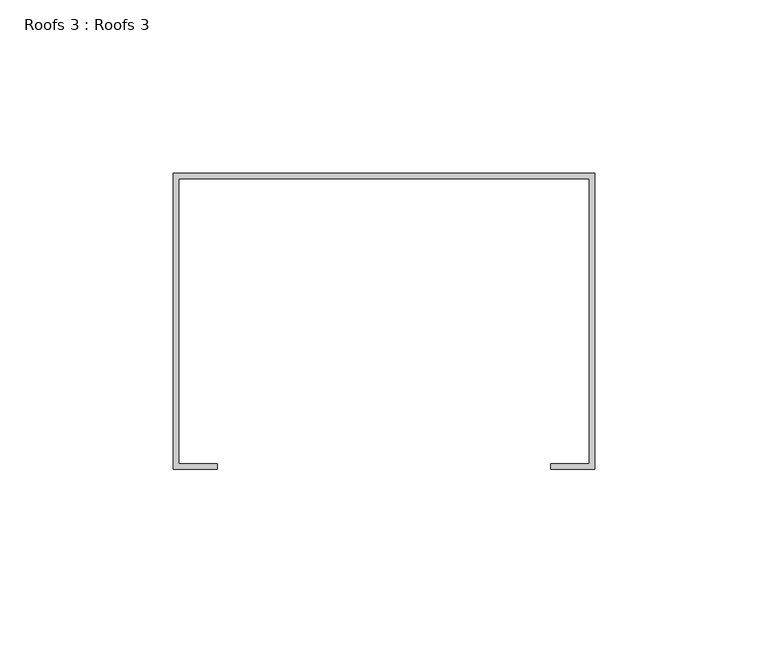
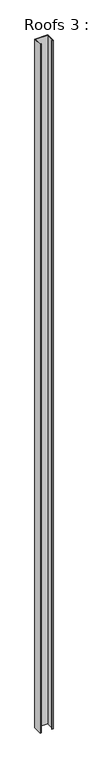
"""IFC4 building model written with IfcOpenShell, lengths in millimetres: proxy geometry, Roofs 3 : Roofs 3."""

from ifc_helpers import new_model, si_unit, frame, origin, place, context, project, spatial, polyline, outline, extrude, source, transform, mapped, element, save


def roofs_3_roofs_3_c517c0f6(model_context):
    return source(origin(), model_context, "Body", "SweptSolid", [
        extrude(outline(polyline([(23391.8090778, 25490.804275), (23391.8090778, 25576.0719112), (23513.2528278, 25576.0719112), (23513.2528278, 25490.804275), (23500.5528278, 25490.804275), (23500.5528278, 25492.391775), (23511.6653278, 25492.391775), (23511.6653278, 25574.4844112), (23393.3965778, 25574.4844112), (23393.3965778, 25492.391775), (23404.5090778, 25492.391775), (23404.5090778, 25490.804275), (23391.8090778, 25490.804275)])), frame((0.0, 0.0, 265354.8970617), z_axis=(0.0, 0.0, 1.0), x_axis=(1.0, 0.0, 0.0)), (0.0, 0.0, 1.0), 6854.6731469),
    ])


if __name__ == "__main__":
    model = new_model("IFC4")
    model_context = context("Model", 3, world=origin())
    ifc_project = project(units=[si_unit("LENGTHUNIT", "METRE", prefix="MILLI")], contexts=[model_context])
    site = spatial("IfcSite", under=ifc_project)
    building = spatial("IfcBuilding", under=site)
    placement = place(None, origin())
    roofs_3_roofs_3_shape = roofs_3_roofs_3_c517c0f6(model_context)
    element("IfcBuildingElementProxy", 1, Name="Roofs 3 : Roofs 3", ObjectType="Roofs 3 : Roofs 3", at=placement, inside=building, context=model_context, shape_type="MappedRepresentation", body=[
        mapped(roofs_3_roofs_3_shape, transform((0.0, 0.0, 0.0), x_axis=(1.0, 0.0, 0.0), y_axis=(0.0, 1.0, 0.0), z_axis=(0.0, 0.0, 1.0))),
    ])
    save(model, "model.ifc")

# Revit data of these elements
# Element 1 (IfcBuildingElementProxy, "Roofs 3 : Roofs 3")
#   Materials on its faces: "OPEN FACED DOWNSPOUT (COLOR: GALVANIZED)"
# Materials
#   "OPEN FACED DOWNSPOUT (COLOR: GALVANIZED)": class "Generic", colour RGB 120 120 120, transparency 0, Cost = 0
